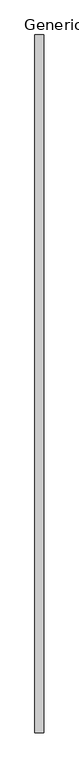
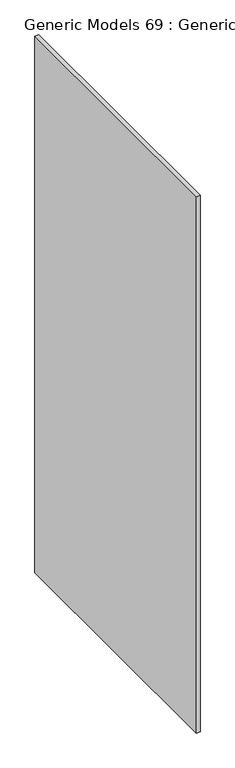
"""IFC4 building model written with IfcOpenShell, lengths in millimetres: proxy geometry, Generic Models 69 : Generic Models 1."""

from ifc_helpers import new_model, si_unit, frame, origin, place, context, project, spatial, polyline, outline, extrude, source, transform, mapped, element, save


def generic_models_69_generic_models_1_75d49a3d(model_context):
    return source(origin(), model_context, "Body", "SweptSolid", [
        extrude(outline(polyline([(50914.3, 1219.2), (50914.3, 0.0), (50898.425, 0.0), (50898.425, 1219.2), (50914.3, 1219.2)])), frame((0.0, 0.0, 3054.35), z_axis=(0.0, 0.0, 1.0), x_axis=(1.0, 0.0, 0.0)), (0.0, 0.0, 1.0), 2472.928125),
    ])


if __name__ == "__main__":
    model = new_model("IFC4")
    model_context = context("Model", 3, world=origin())
    ifc_project = project(units=[si_unit("LENGTHUNIT", "METRE", prefix="MILLI")], contexts=[model_context])
    site = spatial("IfcSite", under=ifc_project)
    building = spatial("IfcBuilding", under=site)
    placement = place(None, origin())
    generic_models_69_generic_models_1_shape = generic_models_69_generic_models_1_75d49a3d(model_context)
    element("IfcBuildingElementProxy", 1, Name="Generic Models 69 : Generic Models 1", ObjectType="Generic Models 69 : Generic Models 1", at=placement, inside=building, context=model_context, shape_type="MappedRepresentation", body=[
        mapped(generic_models_69_generic_models_1_shape, transform((0.0, 0.0, 0.0), x_axis=(1.0, 0.0, 0.0), y_axis=(0.0, 1.0, 0.0), z_axis=(0.0, 0.0, 1.0))),
    ])
    save(model, "model.ifc")

# Revit data of these elements
# Element 1 (IfcBuildingElementProxy, "Generic Models 69 : Generic Models 1")
#   Materials on its faces: "5/8\" GYP. BD"
# Materials
#   "5/8\" GYP. BD": class "Generic", colour RGB 255 255 255, transparency 0, Description = "Gypsum Wall Board", Cost = 0
